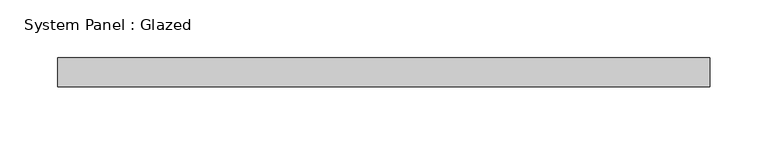
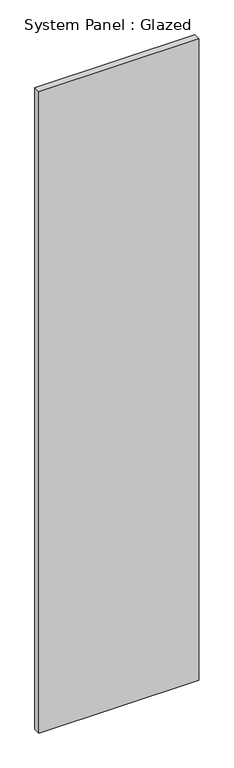
"""IFC4 building model written with IfcOpenShell, lengths in millimetres: plate geometry, System Panel : Glazed."""

from ifc_helpers import new_model, si_unit, origin, origin_with_axes, place, context, project, spatial, polyline, outline, extrude, source, transform, mapped, element, save


def system_panel_glazed_5a3b5b37(model_context):
    return source(origin(), model_context, "Body", "SweptSolid", [
        extrude(outline(polyline([(282.4999998, 24.5), (-282.4999998, 24.5), (-282.4999998, 49.5), (282.4999998, 49.5), (282.4999998, 24.5)])), origin_with_axes(), (0.0, 0.0, 1.0), 2400.0),
    ])


if __name__ == "__main__":
    model = new_model("IFC4")
    model_context = context("Model", 3, world=origin())
    ifc_project = project(units=[si_unit("LENGTHUNIT", "METRE", prefix="MILLI")], contexts=[model_context])
    site = spatial("IfcSite", under=ifc_project)
    building = spatial("IfcBuilding", under=site)
    placement = place(None, origin())
    system_panel_glazed_shape = system_panel_glazed_5a3b5b37(model_context)
    element("IfcPlate", 1, ObjectType="System Panel : Glazed", at=placement, inside=building, context=model_context, shape_type="MappedRepresentation", body=[
        mapped(system_panel_glazed_shape, transform((0.0, 0.0, 0.0), x_axis=(1.0, 0.0, 0.0), y_axis=(0.0, 1.0, 0.0), z_axis=(0.0, 0.0, 1.0))),
    ])
    save(model, "model.ifc")

# Revit data of these elements
# Type "System Panel : Glazed"
#   Keynote = "H11"
#   Construction Type Id = "GSP4R"
#   Analytic Construction = "1/8 in Pilkington single glazing"
#   Visual Light Transmittance = 0.9
#   Solar Heat Gain Coefficient = 0.86
#   Heat Transfer Coefficient (U) = 6.7069 W/(m²·K)
#   Define Thermal Properties by = 1
# Element 1 (IfcPlate, "System Panel : Glazed")
#   Materials on its faces: "Glass"
# Materials
#   "Glass": class "Glass", colour RGB 0 128 192, transparency 0.9, Description = "Soda Lime Glass", Cost = 0
